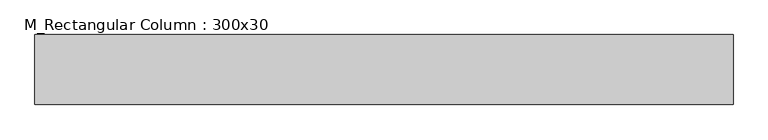
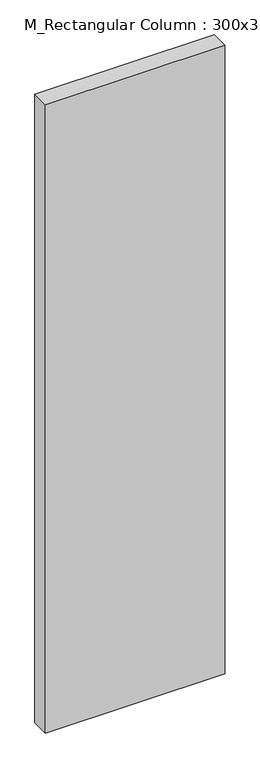
"""IFC4 building model written with IfcOpenShell, lengths in millimetres: column geometry, M_Rectangular Column : 300x30."""

from ifc_helpers import new_model, si_unit, frame, origin, place, context, project, spatial, polyline, outline, extrude, source, transform, mapped, element, save


def m_rectangular_column_300x30_b7aa0491(model_context):
    return source(origin(), model_context, "Body", "SweptSolid", [
        extrude(outline(polyline([(1500.0, 150.0), (1500.0, -150.0), (-1500.0, -150.0), (-1500.0, 150.0), (1500.0, 150.0)])), frame((0.0, 0.0, -3200.0), z_axis=(0.0, 0.0, 1.0), x_axis=(1.0, 0.0, 0.0)), (0.0, 0.0, 1.0), 11100.0),
    ])


if __name__ == "__main__":
    model = new_model("IFC4")
    model_context = context("Model", 3, world=origin())
    ifc_project = project(units=[si_unit("LENGTHUNIT", "METRE", prefix="MILLI")], contexts=[model_context])
    site = spatial("IfcSite", under=ifc_project)
    building = spatial("IfcBuilding", under=site)
    placement = place(None, origin())
    m_rectangular_column_300x30_shape = m_rectangular_column_300x30_b7aa0491(model_context)
    element("IfcColumn", 1, ObjectType="M_Rectangular Column : 300x30", at=placement, inside=building, context=model_context, shape_type="MappedRepresentation", body=[
        mapped(m_rectangular_column_300x30_shape, transform((0.0, 0.0, 0.0), x_axis=(1.0, 0.0, 0.0), y_axis=(0.0, 1.0, 0.0), z_axis=(0.0, 0.0, 1.0))),
    ])
    save(model, "model.ifc")

# Revit data of these elements
# Type "M_Rectangular Column : 300x30"
#   Depth = 30 cm
#   Offset Base = 0 cm
#   Offset Top = 0 cm
#   Width = 300 cm
#   Material = none
